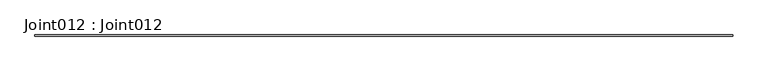
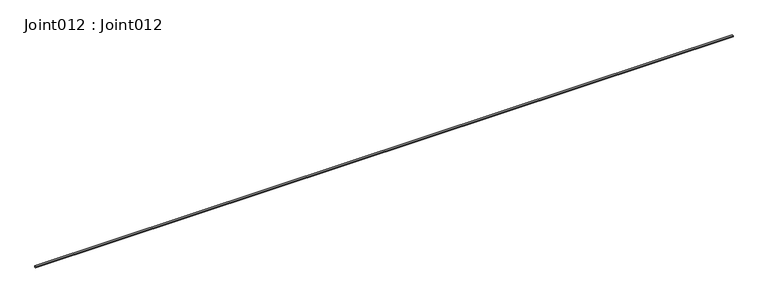
"""IFC4 building model written with IfcOpenShell, lengths in millimetres: proxy geometry, Joint012 : Joint012."""

from ifc_helpers import new_model, si_unit, point, frame, frame_2d, origin, place, context, project, spatial, polyline, circle_curve, trimmed, segment, composite_curve, outline, extrude, source, transform, mapped, element, save


def joint012_joint012_801eaf96(model_context):
    return source(origin(), model_context, "Body", "SweptSolid", [
        extrude(outline(composite_curve([segment(trimmed(circle_curve(frame_2d((-4627.2943844, 38428.99375)), 5.4132205), [point((-4625.6960524, 38423.821875))], [point((-4628.8927164, 38423.821875))], False, "CARTESIAN"), True, "CONTINUOUS"), segment(polyline([(-4628.8927164, 38423.821875), (-4628.8927164, 38427.7398437)]), True, "CONTINUOUS"), segment(trimmed(circle_curve(frame_2d((-4627.2943844, 38432.9117187)), 5.4132205), [point((-4628.8927164, 38427.7398437))], [point((-4625.6960524, 38427.7398437))], True, "CARTESIAN"), True, "CONTINUOUS"), segment(polyline([(-4625.6960524, 38427.7398437), (-4625.6960524, 38423.821875)]), True, "CONTINUOUS")], self_intersect=False)), frame((12383.0178845, 0.0, 0.0), z_axis=(1.0, 0.0, 0.0), x_axis=(0.0, 1.0, 0.0)), (0.0, 0.0, 1.0), 2000.0),
    ])


if __name__ == "__main__":
    model = new_model("IFC4")
    model_context = context("Model", 3, world=origin())
    ifc_project = project(units=[si_unit("LENGTHUNIT", "METRE", prefix="MILLI")], contexts=[model_context])
    site = spatial("IfcSite", under=ifc_project)
    building = spatial("IfcBuilding", under=site)
    placement = place(None, origin())
    joint012_joint012_shape = joint012_joint012_801eaf96(model_context)
    element("IfcBuildingElementProxy", 1, Name="Joint012 : Joint012", ObjectType="Joint012 : Joint012", at=placement, inside=building, context=model_context, shape_type="MappedRepresentation", body=[
        mapped(joint012_joint012_shape, transform((0.0, 0.0, 0.0), x_axis=(1.0, 0.0, 0.0), y_axis=(0.0, 1.0, 0.0), z_axis=(0.0, 0.0, 1.0))),
    ])
    save(model, "model.ifc")

# Revit data of these elements
# Type "Joint012 : Joint012"
#   NameOverride = "Joint012"
# Element 1 (IfcBuildingElementProxy, "Joint012 : Joint012")
#   Materials on its faces: "SILICON JOINT"
# Materials
#   "SILICON JOINT": class "Unassigned", colour RGB 150 184 127, transparency 0
